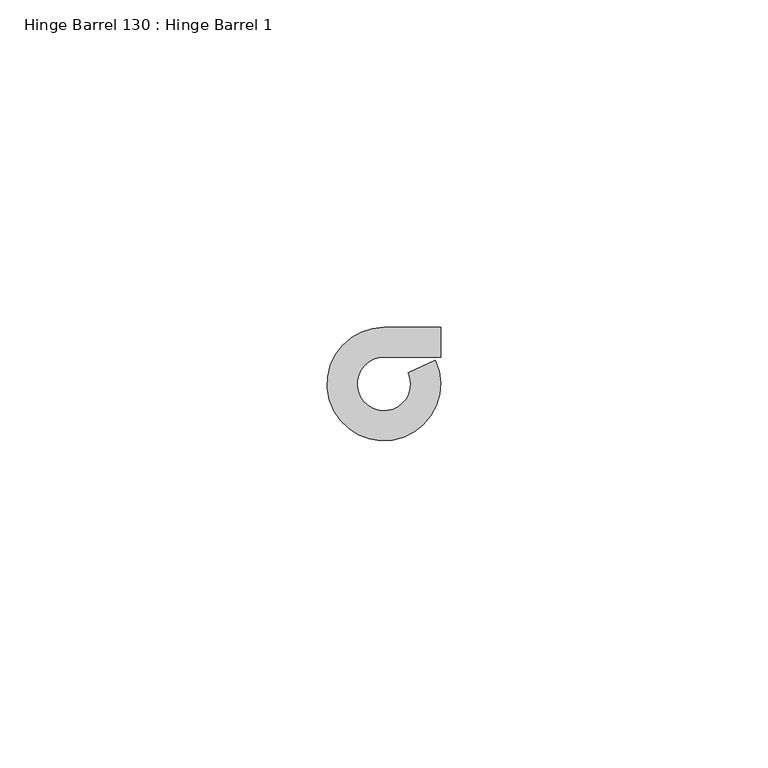
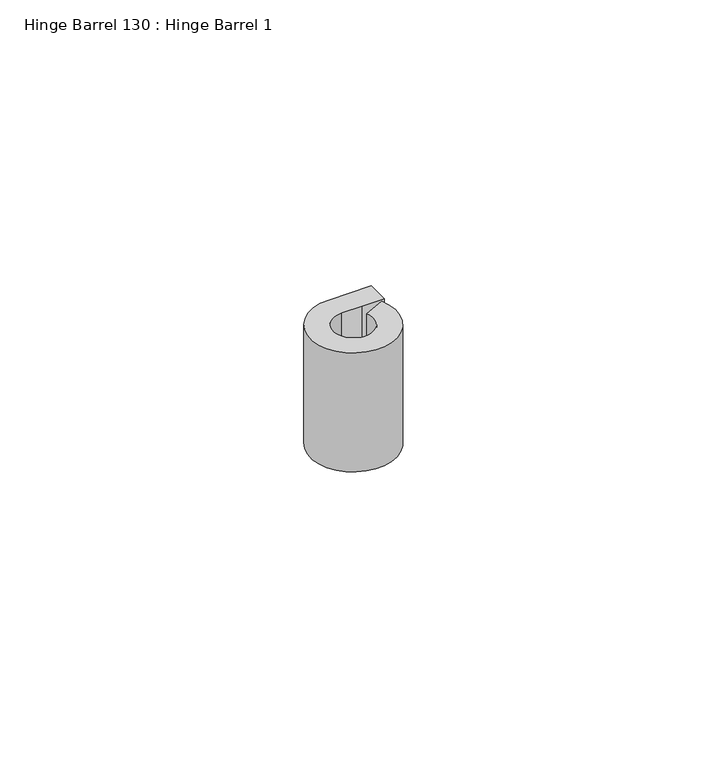
"""IFC4 building model written with IfcOpenShell, lengths in millimetres: proxy geometry, Hinge Barrel 130 : Hinge Barrel 1."""

from ifc_helpers import new_model, si_unit, point, frame, frame_2d, origin, place, context, project, spatial, polyline, circle_curve, trimmed, segment, composite_curve, outline, extrude, source, transform, mapped, element, save


def hinge_barrel_130_hinge_barrel_1_8e11106c(model_context):
    return source(origin(), model_context, "Body", "SweptSolid", [
        extrude(outline(composite_curve([segment(polyline([(587323.2214739, -536306.2758841), (587319.1320739, -536306.2758841)]), True, "CONTINUOUS"), segment(trimmed(circle_curve(frame_2d((587319.1320739, -536310.3652841)), 4.0894), [point((587319.1320739, -536306.2758841))], [point((587322.8436736, -536308.6485371))], True, "CARTESIAN"), True, "CONTINUOUS"), segment(polyline([(587322.8436736, -536308.6485371), (587326.986084, -536306.7325249)]), True, "CONTINUOUS"), segment(trimmed(circle_curve(frame_2d((587319.1320739, -536310.3652841)), 8.6534625), [point((587326.986084, -536306.7325249))], [point((587319.1320739, -536301.7118216))], False, "CARTESIAN"), True, "CONTINUOUS"), segment(polyline([(587319.1320739, -536301.7118216), (587327.7934739, -536301.7118216), (587327.7934739, -536306.2758841), (587323.2214739, -536306.2758841)]), True, "CONTINUOUS")], self_intersect=False)), frame((0.0, 0.0, 412.75), z_axis=(0.0, 0.0, 1.0), x_axis=(1.0, 0.0, 0.0)), (0.0, 0.0, 1.0), 25.4),
    ])


if __name__ == "__main__":
    model = new_model("IFC4")
    model_context = context("Model", 3, world=origin())
    ifc_project = project(units=[si_unit("LENGTHUNIT", "METRE", prefix="MILLI")], contexts=[model_context])
    site = spatial("IfcSite", under=ifc_project)
    building = spatial("IfcBuilding", under=site)
    placement = place(None, origin())
    hinge_barrel_130_hinge_barrel_1_shape = hinge_barrel_130_hinge_barrel_1_8e11106c(model_context)
    element("IfcBuildingElementProxy", 1, Name="Hinge Barrel 130 : Hinge Barrel 1", ObjectType="Hinge Barrel 130 : Hinge Barrel 1", at=placement, inside=building, context=model_context, shape_type="MappedRepresentation", body=[
        mapped(hinge_barrel_130_hinge_barrel_1_shape, transform((0.0, 0.0, 0.0), x_axis=(1.0, 0.0, 0.0), y_axis=(0.0, 1.0, 0.0), z_axis=(0.0, 0.0, 1.0))),
    ])
    save(model, "model.ifc")

# Revit data of these elements
# Element 1 (IfcBuildingElementProxy, "Hinge Barrel 130 : Hinge Barrel 1")
#   Materials on its faces: "6\"X6\" WELD-ON STL BUTT HINGE"
# Materials
#   "6\"X6\" WELD-ON STL BUTT HINGE": class "Metal", colour RGB 189 187 185, transparency 0, Description = "Carbon steel", Cost = 0
